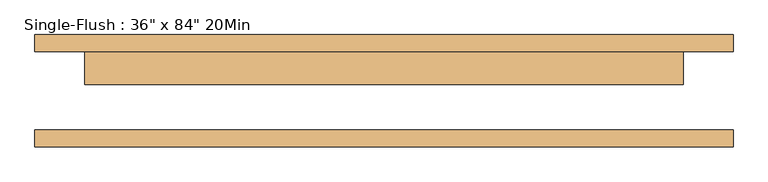
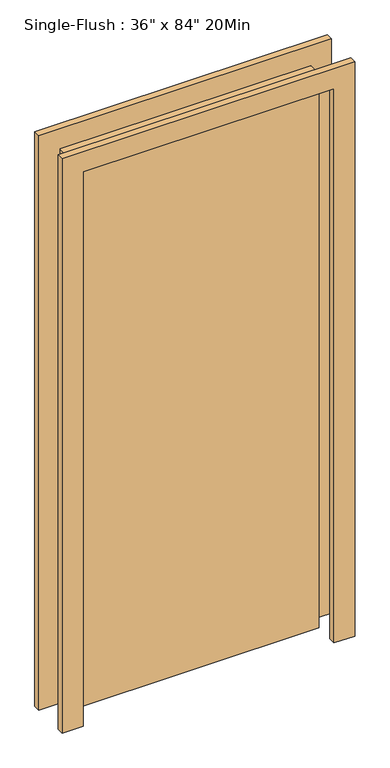
"""IFC4 building model written with IfcOpenShell, lengths in millimetres: door geometry."""

from ifc_helpers import new_model, si_unit, frame, origin, origin_with_axes, place, context, project, spatial, polyline, outline, extrude, source, transform, mapped, element, save


def door_aa02eb04(model_context):
    return source(origin(), model_context, "Body", "SweptSolid", [
        extrude(outline(polyline([(2209.8, -533.4), (0.0, -533.4), (0.0, -457.2), (2133.6, -457.2), (2133.6, 457.2), (0.0, 457.2), (0.0, 533.4), (2209.8, 533.4), (2209.8, -533.4)])), frame((0.0, 60.325, 0.0), z_axis=(0.0, 1.0, 0.0), x_axis=(0.0, 0.0, 1.0)), (0.0, 0.0, 1.0), 25.4),
        extrude(outline(polyline([(2209.8, 533.4), (2209.8, -533.4), (0.0, -533.4), (0.0, -457.2), (2133.6, -457.2), (2133.6, 457.2), (0.0, 457.2), (0.0, 533.4), (2209.8, 533.4)])), frame((0.0, -85.725, 0.0), z_axis=(0.0, 1.0, 0.0), x_axis=(0.0, 0.0, 1.0)), (0.0, 0.0, 1.0), 25.4),
        extrude(outline(polyline([(457.2, 9.525), (-457.2, 9.525), (-457.2, 60.325), (457.2, 60.325), (457.2, 9.525)])), origin_with_axes(), (0.0, 0.0, 1.0), 2133.6),
    ])


if __name__ == "__main__":
    model = new_model("IFC4")
    model_context = context("Model", 3, world=origin())
    ifc_project = project(units=[si_unit("LENGTHUNIT", "METRE", prefix="MILLI")], contexts=[model_context])
    site = spatial("IfcSite", under=ifc_project)
    building = spatial("IfcBuilding", under=site)
    placement = place(None, origin())
    door_shape = door_aa02eb04(model_context)
    element("IfcDoor", 1, ObjectType="Single-Flush : 36\" x 84\" 20Min", at=placement, inside=building, context=model_context, shape_type="MappedRepresentation", body=[
        mapped(door_shape, transform((0.0, 0.0, 0.0), x_axis=(1.0, 0.0, 0.0), y_axis=(0.0, 1.0, 0.0), z_axis=(0.0, 0.0, 1.0))),
    ])
    save(model, "model.ifc")

# Revit data of these elements
# Type "Single-Flush : 36\" x 84\" 20Min"
#   Type Mark = "23"
#   Fire Rating = "20 Min."
#   Assembly Code = "C1020"
#   Thickness = 50.8 mm
#   Height = 2133.6 mm
#   Trim Projection Ext = 25.4 mm
#   Trim Projection Int = 25.4 mm
#   Trim Width = 76.2 mm
#   Width = 914.4 mm
#   Define Thermal Properties by = 0
#   Door Material = Door - Panel
#   Frame Material = Door - Frame
#   Function = (empty or 0)
#   Wall Closure = (empty or 0)
# Element 1 (IfcDoor, "Single-Flush : 36\" x 84\" 20Min")
#   Materials on its faces: "Door - Frame", "Door - Panel"
# Materials
#   "Door - Panel": class "Wood", colour RGB 210 159 95, transparency 0, Cost = 0
#   "Door - Frame": class "Miscellaneous", colour RGB 118 70 51, transparency 0, Cost = 0
